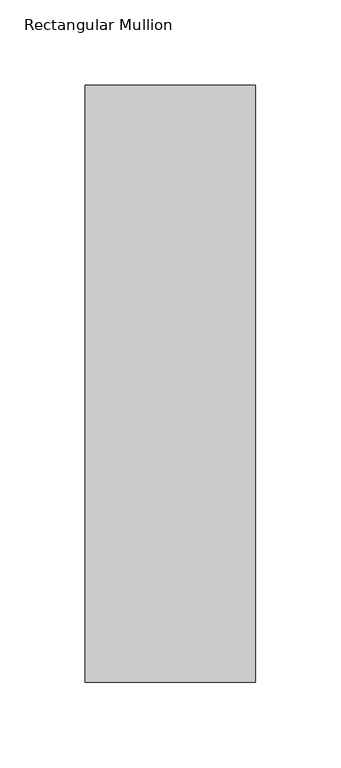
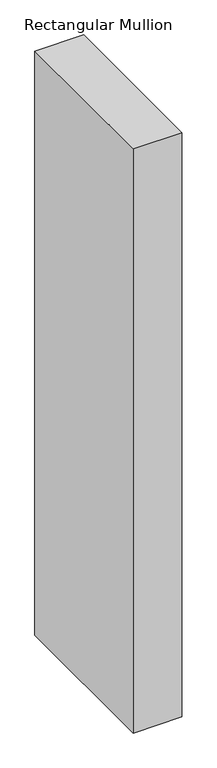
"""IFC4 building model written with IfcOpenShell, lengths in millimetres: member geometry, Rectangular Mullion : WWm-100x350-100mmOffset."""

from ifc_helpers import new_model, si_unit, frame, origin, place, context, project, spatial, polyline, outline, extrude, source, transform, mapped, element, save


def rectangular_mullion_cd50211b(model_context):
    return source(origin(), model_context, "Body", "SweptSolid", [
        extrude(outline(polyline([(0.0, 175.0), (0.0, -175.0), (-100.0, -175.0), (-100.0, 175.0), (0.0, 175.0)])), frame((0.0, 0.0, -1269.0), z_axis=(0.0, 0.0, 1.0), x_axis=(1.0, 0.0, 0.0)), (0.0, 0.0, 1.0), 1269.0),
    ])


if __name__ == "__main__":
    model = new_model("IFC4")
    model_context = context("Model", 3, world=origin())
    ifc_project = project(units=[si_unit("LENGTHUNIT", "METRE", prefix="MILLI")], contexts=[model_context])
    site = spatial("IfcSite", under=ifc_project)
    building = spatial("IfcBuilding", under=site)
    placement = place(None, origin())
    rectangular_mullion_shape = rectangular_mullion_cd50211b(model_context)
    element("IfcMember", 1, ObjectType="Rectangular Mullion : WWm-100x350-100mmOffset", at=placement, inside=building, context=model_context, shape_type="MappedRepresentation", body=[
        mapped(rectangular_mullion_shape, transform((0.0, 0.0, 0.0), x_axis=(1.0, 0.0, 0.0), y_axis=(0.0, 1.0, 0.0), z_axis=(0.0, 0.0, 1.0))),
    ])
    save(model, "model.ifc")

# Revit data of these elements
# Type "Rectangular Mullion : WWm-100x350-100mmOffset"
#   built-in parameter 1007304 = 1.14829 (stored number, unit not read)
#   built-in parameter 1007301 = 0.164042 (stored number, unit not read)
#   built-in parameter 1007300 = 0.164042 (stored number, unit not read)
# Element 1 (IfcMember, "Rectangular Mullion : WWm-100x350-100mmOffset")
#   Materials on its faces: "WW-EC-RGB-Mullion"
# Materials
#   "WW-EC-RGB-Mullion": class "Generic", colour RGB 255 255 255, transparency 0, Comments = "If region requests black mullions, switch asset color to RGB 25-25-25", Description = "Generic Color", Cost = 0
